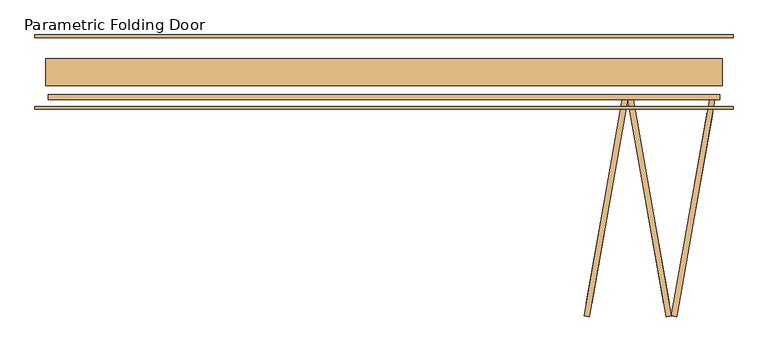
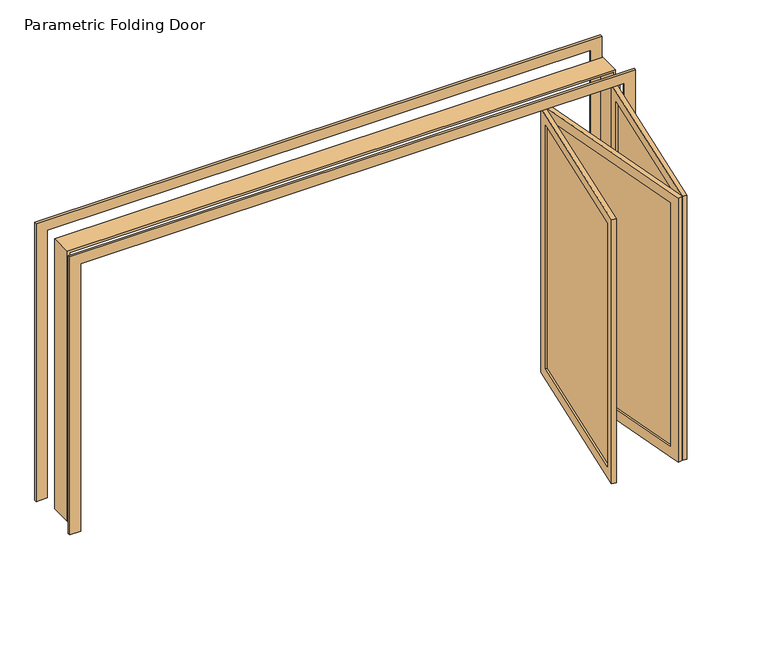
"""IFC4 building model written with IfcOpenShell, lengths in millimetres: door geometry, Parametric Folding Door : Bifold door [parametric]."""

from ifc_helpers import new_model, si_unit, frame, origin, place, context, project, spatial, polyline, outline, extrude, source, transform, mapped, element, save


def parametric_folding_door_a182b64b(model_context):
    return source(origin(), model_context, "Body", "SweptSolid", [
        extrude(outline(polyline([(1445.5871901, -529.3818366), (1449.5264211, -530.0764294), (1198.894218, -1951.4822862), (1194.954987, -1950.7876935), (1445.5871901, -529.3818366)])), frame((0.0, 0.0, 100.0), z_axis=(0.0, 0.0, 1.0), x_axis=(1.0, 0.0, 0.0)), (0.0, 0.0, 1.0), 2365.0),
        extrude(outline(polyline([(0.0, -1643.3333333), (0.0, 0.0), (2565.0, 0.0), (2565.0, -1643.3333333), (0.0, -1643.3333333)]), holes=[polyline([(2465.0, -1543.3333333), (2465.0, -100.0), (100.0, -100.0), (100.0, -1543.3333333), (2465.0, -1543.3333333)])]), frame((1484.6177784, -434.7213213, 0.0), z_axis=(-0.9848077530122078, 0.17364817766693175, 0.0), x_axis=(0.0, 0.0, 1.0)), (0.0, 0.0, 1.0), 40.0),
        extrude(outline(polyline([(1523.6483668, -529.3818366), (1774.2805699, -1950.7876935), (1770.3413389, -1951.4822862), (1519.7091358, -530.0764294), (1523.6483668, -529.3818366)])), frame((0.0, 0.0, 100.0), z_axis=(0.0, 0.0, 1.0), x_axis=(1.0, 0.0, 0.0)), (0.0, 0.0, 1.0), 2365.0),
        extrude(outline(polyline([(0.0, 1643.3333333), (2565.0, 1643.3333333), (2565.0, 0.0), (0.0, 0.0), (0.0, 1643.3333333)]), holes=[polyline([(2465.0, 1543.3333333), (100.0, 1543.3333333), (100.0, 100.0), (2465.0, 100.0), (2465.0, 1543.3333333)])]), frame((1484.6177784, -434.7213213, 0.0), z_axis=(0.9848077530122078, 0.17364817766693175, 0.0), x_axis=(0.0, 0.0, 1.0)), (0.0, 0.0, 1.0), 40.0),
        extrude(outline(polyline([(2095.0954876, -529.3818366), (2099.0347186, -530.0764294), (1848.4025155, -1951.4822862), (1844.4632845, -1950.7876935), (2095.0954876, -529.3818366)])), frame((0.0, 0.0, 100.0), z_axis=(0.0, 0.0, 1.0), x_axis=(1.0, 0.0, 0.0)), (0.0, 0.0, 1.0), 2365.0),
        extrude(outline(polyline([(0.0, -1643.3333333), (0.0, 0.0), (2565.0, 0.0), (2565.0, -1643.3333333), (0.0, -1643.3333333)]), holes=[polyline([(2465.0, -1543.3333333), (2465.0, -100.0), (100.0, -100.0), (100.0, -1543.3333333), (2465.0, -1543.3333333)])]), frame((2134.1260759, -434.7213213, 0.0), z_axis=(-0.9848077530122078, 0.17364817766693175, 0.0), x_axis=(0.0, 0.0, 1.0)), (0.0, 0.0, 1.0), 40.0),
        extrude(outline(polyline([(2700.0, -2930.8739241), (0.0, -2930.8739241), (0.0, -2830.8739241), (2600.0, -2830.8739241), (2600.0, 2169.1260759), (0.0, 2169.1260759), (0.0, 2269.1260759), (2700.0, 2269.1260759), (2700.0, -2930.8739241)])), frame((0.0, 29.7786788, 0.0), z_axis=(0.0, 1.0, 0.0), x_axis=(0.0, 0.0, 1.0)), (0.0, 0.0, 1.0), 20.0),
        extrude(outline(polyline([(2600.0, -2830.8739241), (2600.0, 2169.1260759), (0.0, 2169.1260759), (0.0, 2269.1260759), (2700.0, 2269.1260759), (2700.0, -2930.8739241), (0.0, -2930.8739241), (0.0, -2830.8739241), (2600.0, -2830.8739241)])), frame((0.0, -504.7213212, 0.0), z_axis=(0.0, 1.0, 0.0), x_axis=(0.0, 0.0, 1.0)), (0.0, 0.0, 1.0), 20.0),
        extrude(outline(polyline([(0.0, 2169.1260759), (0.0, 2189.1260759), (2620.0, 2189.1260759), (2620.0, -2850.8739241), (0.0, -2850.8739241), (0.0, -2830.8739241), (2600.0, -2830.8739241), (2600.0, 2169.1260759), (0.0, 2169.1260759)])), frame((0.0, -327.4713212, 0.0), z_axis=(0.0, 1.0, 0.0), x_axis=(0.0, 0.0, 1.0)), (0.0, 0.0, 1.0), 200.0),
        extrude(outline(polyline([(0.0, 2134.1260759), (0.0, 2169.1260759), (2600.0, 2169.1260759), (2600.0, -2830.8739241), (0.0, -2830.8739241), (0.0, -2795.8739241), (2565.0, -2795.8739241), (2565.0, 2134.1260759), (0.0, 2134.1260759)])), frame((0.0, -434.7213213, 0.0), z_axis=(0.0, 1.0, 0.0), x_axis=(0.0, 0.0, 1.0)), (0.0, 0.0, 1.0), 40.0),
    ])


if __name__ == "__main__":
    model = new_model("IFC4")
    model_context = context("Model", 3, world=origin())
    ifc_project = project(units=[si_unit("LENGTHUNIT", "METRE", prefix="MILLI")], contexts=[model_context])
    site = spatial("IfcSite", under=ifc_project)
    building = spatial("IfcBuilding", under=site)
    placement = place(None, origin())
    parametric_folding_door_shape = parametric_folding_door_a182b64b(model_context)
    element("IfcDoor", 1, ObjectType="Parametric Folding Door : Bifold door [parametric]", at=placement, inside=building, context=model_context, shape_type="MappedRepresentation", body=[
        mapped(parametric_folding_door_shape, transform((0.0, 0.0, 0.0), x_axis=(1.0, 0.0, 0.0), y_axis=(0.0, 1.0, 0.0), z_axis=(0.0, 0.0, 1.0))),
    ])
    save(model, "model.ifc")

# Revit data of these elements
# Type "Parametric Folding Door : Bifold door [parametric]"
#   Type Mark = "52"
#   Analytic Construction = "<None>"
#   Trail width = 35 mm
#   Trail thickness = 40 mm
#   Rough Width = 5040 mm
#   Rough Height = 5020 mm
#   Panel width = 1643.333 mm
#   Panel thickness = 40 mm
#   Panel space = 324.754 mm
#   Panel mullion width = 100 mm
#   Panel height = 2565 mm
#   Open angle = 80.00°
#   Jamb width = 200 mm
#   Jamb thickness = 20 mm
#   Glass thickness = 4 mm
#   Frame thickness = 20 mm
#   Frame Width = 100 mm
#   Height = 2600 mm
#   Width = 5000 mm
#   External offset = 50 mm
#   Right 5 = no
#   Right 4 = no
#   Right 3 = no
#   Right 2 = no
#   Right 1 = no
#   No of right panels = 0
#   No of left panels = 3
#   Left 5 = no
#   Left 4 = no
#   Left 3 = yes
#   Left 2 = yes
#   Left 1 = yes
#   Internal frame visible = yes
#   Function = 1
#   Wall Closure = 4
#   External frame visible = yes
#   Define Thermal Properties by = 1
#   Trail = Door - Bifold - Jamb & Trail
#   Panel mullion = Door - Bifold - Panel Mullion
#   Jamb = Door - Bifold - Jamb & Trail
#   Glass = Door - Bifold - Glass
#   Assembly Code = ""
# Element 1 (IfcDoor, "Parametric Folding Door : Bifold door [parametric]")
#   Materials on its faces: "Door - Bifold - Jamb & Trail", "Door - Bifold - Panel Mullion", "Door - Bifold - Glass"
# Materials
#   "Door - Bifold - Jamb & Trail": class "Metal", colour RGB 0 0 0, transparency 0
#   "Door - Bifold - Panel Mullion": class "Metal", colour RGB 0 0 0, transparency 0, Cost = 0
#   "Door - Bifold - Glass": class "Glass", colour RGB 165 165 165, transparency 0.95
